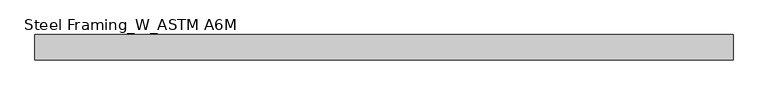
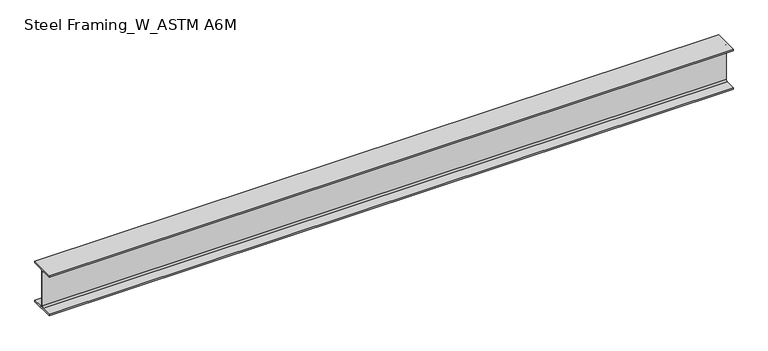
"""IFC4 building model written with IfcOpenShell, lengths in millimetres: beam geometry, Steel Framing_W_ASTM A6M : H_SB_ASB_W360x64."""

from ifc_helpers import new_model, si_unit, point, frame, frame_2d, origin, place, context, project, spatial, polyline, circle_curve, trimmed, segment, composite_curve, outline, extrude, source, transform, mapped, element, save


def steel_framing_w_astm_a6m_8cc9ac01(model_context):
    return source(origin(), model_context, "Body", "SweptSolid", [
        extrude(outline(composite_curve([segment(polyline([(101.5, -160.5), (101.5, -174.0), (-101.5, -174.0), (-101.5, -160.5), (-18.775, -160.5)]), True, "CONTINUOUS"), segment(trimmed(circle_curve(frame_2d((-18.775, -145.6)), 14.9), [point((-18.775, -160.5))], [point((-3.875, -145.6))], True, "CARTESIAN"), True, "CONTINUOUS"), segment(polyline([(-3.875, -145.6), (-3.875, 145.6)]), True, "CONTINUOUS"), segment(trimmed(circle_curve(frame_2d((-18.775, 145.6)), 14.9), [point((-3.875, 145.6))], [point((-18.775, 160.5))], True, "CARTESIAN"), True, "CONTINUOUS"), segment(polyline([(-18.775, 160.5), (-101.5, 160.5), (-101.5, 174.0), (101.5, 174.0), (101.5, 160.5), (18.775, 160.5)]), True, "CONTINUOUS"), segment(trimmed(circle_curve(frame_2d((18.775, 145.6)), 14.9), [point((18.775, 160.5))], [point((3.875, 145.6))], True, "CARTESIAN"), True, "CONTINUOUS"), segment(polyline([(3.875, 145.6), (3.875, -145.6)]), True, "CONTINUOUS"), segment(trimmed(circle_curve(frame_2d((18.775, -145.6)), 14.9), [point((3.875, -145.6))], [point((18.775, -160.5))], True, "CARTESIAN"), True, "CONTINUOUS"), segment(polyline([(18.775, -160.5), (101.5, -160.5)]), True, "CONTINUOUS")], self_intersect=False)), frame((-2696.5, 0.0, 0.0), z_axis=(1.0, 0.0, 0.0), x_axis=(0.0, 1.0, 0.0)), (0.0, 0.0, 1.0), 5596.6),
    ])


if __name__ == "__main__":
    model = new_model("IFC4")
    model_context = context("Model", 3, world=origin())
    ifc_project = project(units=[si_unit("LENGTHUNIT", "METRE", prefix="MILLI")], contexts=[model_context])
    site = spatial("IfcSite", under=ifc_project)
    building = spatial("IfcBuilding", under=site)
    placement = place(None, origin())
    steel_framing_w_astm_a6m_shape = steel_framing_w_astm_a6m_8cc9ac01(model_context)
    element("IfcBeam", 1, ObjectType="Steel Framing_W_ASTM A6M : H_SB_ASB_W360x64", at=placement, inside=building, context=model_context, shape_type="MappedRepresentation", body=[
        mapped(steel_framing_w_astm_a6m_shape, transform((0.0, 0.0, 0.0), x_axis=(1.0, 0.0, 0.0), y_axis=(0.0, 1.0, 0.0), z_axis=(0.0, 0.0, 1.0))),
    ])
    save(model, "model.ifc")

# Revit data of these elements
# Type "Steel Framing_W_ASTM A6M : H_SB_ASB_W360x64"
#   Section Name Key = "W14x43"
#   Width = 20.3 cm
#   Web Thickness = 0.775 cm
#   Web Fillet = 1.49 cm
#   Warping Constant = 524000.0 cm⁶
#   Torsional Moment of Inertia = 43.70 cm⁴
#   Section Area = 81.3 cm²
#   Plastic Modulus weak axis = 283.0 cm³
#   Plastic Modulus strong axis = 1140.0 cm³
#   Perimeter = 1.47 m²/m
#   Nominal Weight = 64.00 kgf/m
#   Moment of Inertia weak axis = 1880.00 cm⁴
#   Moment of Inertia strong axis = 17800.00 cm⁴
#   Height = 34.8 cm
#   Flange Thickness = 1.35 cm
#   Elastic Modulus weak axis = 185.0 cm³
#   Elastic Modulus strong axis = 1030.0 cm³
#   Centroid Vertical = 17.4 cm
#   Centroid Horizontal = 10.15 cm
#   Length [instance default] = 1500.000 mm
#   Structural Material [instance default] = Steel, 45-345
#   Bolt Spacing = 0
#   Assembly Code = ""
# Element 1 (IfcBeam, "Steel Framing_W_ASTM A6M : H_SB_ASB_W360x64")
#   Materials on its faces: "Steel, 45-345"
# Materials
#   "Steel, 45-345": class "Metal", colour RGB 189 187 185, transparency 0, Description = "Steel 345 MPa", Cost = 0
